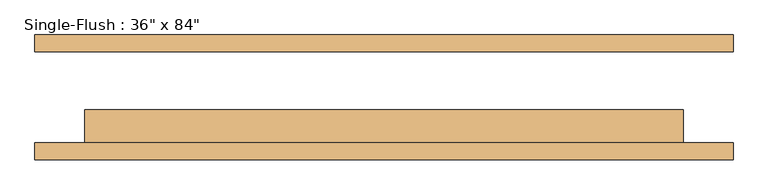
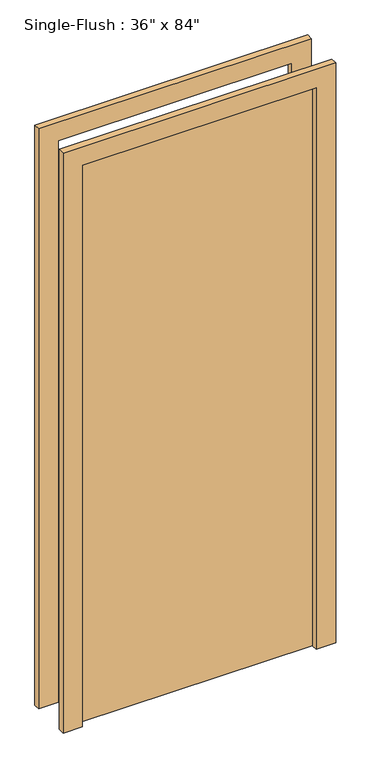
"""IFC4 building model written with IfcOpenShell, lengths in millimetres: door geometry."""

from ifc_helpers import new_model, si_unit, frame, origin, origin_with_axes, place, context, project, spatial, polyline, outline, extrude, source, transform, mapped, element, save


def door_e2a44dfe(model_context):
    return source(origin(), model_context, "Body", "SweptSolid", [
        extrude(outline(polyline([(2399.6, -533.4), (0.0, -533.4), (0.0, -457.2), (2323.4, -457.2), (2323.4, 457.2), (0.0, 457.2), (0.0, 533.4), (2399.6, 533.4), (2399.6, -533.4)])), frame((0.0, -95.25, 0.0), z_axis=(0.0, 1.0, 0.0), x_axis=(0.0, 0.0, 1.0)), (0.0, 0.0, 1.0), 25.4),
        extrude(outline(polyline([(2399.6, 533.4), (2399.6, -533.4), (0.0, -533.4), (0.0, -457.2), (2323.4, -457.2), (2323.4, 457.2), (0.0, 457.2), (0.0, 533.4), (2399.6, 533.4)])), frame((0.0, 69.85, 0.0), z_axis=(0.0, 1.0, 0.0), x_axis=(0.0, 0.0, 1.0)), (0.0, 0.0, 1.0), 25.4),
        extrude(outline(polyline([(457.2, -19.05), (457.2, -69.85), (-457.2, -69.85), (-457.2, -19.05), (457.2, -19.05)])), origin_with_axes(), (0.0, 0.0, 1.0), 2323.4),
    ])


if __name__ == "__main__":
    model = new_model("IFC4")
    model_context = context("Model", 3, world=origin())
    ifc_project = project(units=[si_unit("LENGTHUNIT", "METRE", prefix="MILLI")], contexts=[model_context])
    site = spatial("IfcSite", under=ifc_project)
    building = spatial("IfcBuilding", under=site)
    placement = place(None, origin())
    door_shape = door_e2a44dfe(model_context)
    element("IfcDoor", 1, ObjectType="Single-Flush : 36\" x 84\"", at=placement, inside=building, context=model_context, shape_type="MappedRepresentation", body=[
        mapped(door_shape, transform((0.0, 0.0, 0.0), x_axis=(1.0, 0.0, 0.0), y_axis=(0.0, 1.0, 0.0), z_axis=(0.0, 0.0, 1.0))),
    ])
    save(model, "model.ifc")

# Revit data of these elements
# Type "Single-Flush : 36\" x 84\""
#   Type Mark = "D2"
#   Construction Type Id = "MDOOR"
#   Assembly Code = "C1020"
#   Analytic Construction = "Metal"
#   Thickness = 50.8 mm
#   Heat Transfer Coefficient (U) = 3.7021 W/(m²·K)
#   Height = 2323.4 mm
#   Trim Projection Ext = 25.4 mm
#   Trim Projection Int = 25.4 mm
#   Trim Width = 76.2 mm
#   Width = 914.4 mm
#   Define Thermal Properties by = 1
#   Door Material = wooden-3
#   Frame Material = wooden-3
#   Visual Light Transmittance = 0
#   Solar Heat Gain Coefficient = 0
#   Function = (empty or 0)
#   Wall Closure = (empty or 0)
# Element 1 (IfcDoor, "Single-Flush : 36\" x 84\"")
#   Materials on its faces: "wooden-3"
# Materials
#   "wooden-3": class "Generic", colour RGB 120 120 120, transparency 0, Cost = 0
